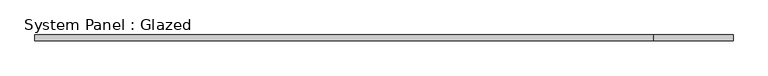
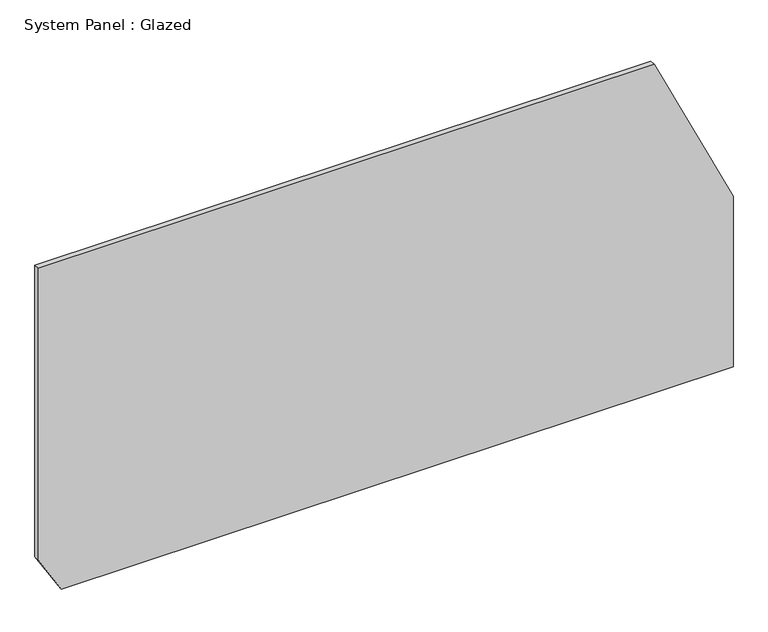
"""IFC4 building model written with IfcOpenShell, lengths in millimetres: plate geometry, System Panel : Glazed."""

import ifcopenshell
import ifcopenshell.guid

model = None  # the IFC model being written
_history = None  # IfcOwnerHistory: only IFC2X3 demands one
_inside = {}  # id of a spatial element -> (the spatial element, [elements in it])
_under = {}  # id of a project, library or spatial element -> (it, [spatial elements below it])
_declared = {}  # id of a project -> (the project, [libraries it declares])
_typed = {}  # id of a type object -> (the type object, [elements of that type])
_made_of = {}  # id of a material, layer set ... -> (it, [elements and type objects made of it])


def new_model(schema):
    """Start an empty IFC model of exactly this schema.

    Asked for "IFC4X3", IfcOpenShell would pick the latest addendum, in which some entities
    have other attributes; the version numbers below select the first issue.
    IFC2X3 requires an IfcOwnerHistory on every rooted entity: one is made here for all.
    """
    global model, _history
    if schema == "IFC4X3":
        model = ifcopenshell.file(schema_version=(4, 3, 0, 0))
    else:
        model = ifcopenshell.file(schema=schema)
    _inside.clear()
    _under.clear()
    _declared.clear()
    _typed.clear()
    _made_of.clear()
    _history = None
    if model.schema == "IFC2X3":
        org = make("IfcOrganization", Name="unknown")
        user = make(
            "IfcPersonAndOrganization",
            ThePerson=make("IfcPerson", FamilyName="unknown"),
            TheOrganization=org,
        )
        app = make(
            "IfcApplication",
            ApplicationDeveloper=org,
            Version="unknown",
            ApplicationFullName="unknown",
            ApplicationIdentifier="unknown",
        )
        _history = make(
            "IfcOwnerHistory",
            OwningUser=user,
            OwningApplication=app,
            ChangeAction="ADDED",
            CreationDate=0,
        )
    return model


def make(cls, **values):
    """One entity of the class cls with the attributes given. An attribute that is None is left unset."""
    return model.create_entity(
        cls, **{name: value for name, value in values.items() if value is not None}
    )


def rooted(cls, **values):
    """An entity with a GlobalId (a new one), such as an element, a storey or a relation."""
    return make(cls, GlobalId=ifcopenshell.guid.new(), OwnerHistory=_history, **values)


def si_unit(unit_type, name, prefix=None):
    """IfcSIUnit, for example si_unit("LENGTHUNIT", "METRE", prefix="MILLI")."""
    return make("IfcSIUnit", UnitType=unit_type, Prefix=prefix, Name=name)


def assignment(units):
    """IfcUnitAssignment: the units of a project."""
    return None if units is None else make("IfcUnitAssignment", Units=units)


def point(xyz):
    """IfcCartesianPoint."""
    return None if xyz is None else make("IfcCartesianPoint", Coordinates=xyz)


def direction(xyz):
    """IfcDirection."""
    return None if xyz is None else make("IfcDirection", DirectionRatios=xyz)


def frame(location, z_axis=None, x_axis=None):
    """IfcAxis2Placement3D, a coordinate frame: its origin and axes. An axis left out is left unset."""
    return make(
        "IfcAxis2Placement3D",
        Location=point(location),
        Axis=direction(z_axis),
        RefDirection=direction(x_axis),
    )


def origin():
    """The frame at (0, 0, 0) with its axes left unset."""
    return frame((0.0, 0.0, 0.0))


def place(relative_to, where):
    """IfcLocalPlacement: puts the frame where relative to a parent placement (None: the world)."""
    return make(
        "IfcLocalPlacement", PlacementRelTo=relative_to, RelativePlacement=where
    )


def context(
    kind, dimensions, precision=None, world=None, true_north=None, identifier=None
):
    """IfcGeometricRepresentationContext, for example the 3D "Model" context."""
    return make(
        "IfcGeometricRepresentationContext",
        ContextIdentifier=identifier,
        ContextType=kind,
        CoordinateSpaceDimension=dimensions,
        Precision=precision,
        WorldCoordinateSystem=world,
        TrueNorth=true_north,
    )


def project(units=None, contexts=None):
    """IfcProject with its units and contexts."""
    return rooted(
        "IfcProject",
        Name="project",
        RepresentationContexts=contexts,
        UnitsInContext=assignment(units),
    )


def spatial(cls, under=None, at=None, **own):
    """A site, building, storey or space (cls), placed at a placement, below another one or the project."""
    s = rooted(cls, ObjectPlacement=at, **own)
    if under is not None:
        _under.setdefault(under.id(), (under, []))[1].append(s)
    return s


def polyline(points):
    """IfcPolyline through the points."""
    return make("IfcPolyline", Points=[point(p) for p in points])


def outline(outer, holes=None, kind="AREA"):
    """IfcArbitraryClosedProfileDef: a profile drawn as a closed curve; with holes, ...WithVoids."""
    if holes is None:
        return make("IfcArbitraryClosedProfileDef", ProfileType=kind, OuterCurve=outer)
    return make(
        "IfcArbitraryProfileDefWithVoids",
        ProfileType=kind,
        OuterCurve=outer,
        InnerCurves=holes,
    )


def extrude(swept, where, along, depth):
    """IfcExtrudedAreaSolid: the profile swept, set in the frame where, extruded along a direction by depth."""
    return make(
        "IfcExtrudedAreaSolid",
        SweptArea=swept,
        Position=where,
        ExtrudedDirection=direction(along),
        Depth=depth,
    )


def shape(context_of_items, identifier, shape_type, items):
    """IfcShapeRepresentation: the items that make up one representation, for example the "Body"."""
    return make(
        "IfcShapeRepresentation",
        ContextOfItems=context_of_items,
        RepresentationIdentifier=identifier,
        RepresentationType=shape_type,
        Items=items,
    )


def source(mapping_origin, context_of_items, identifier, shape_type, items):
    """IfcRepresentationMap: a shape defined once, which mapped items show again and again."""
    return make(
        "IfcRepresentationMap",
        MappingOrigin=mapping_origin,
        MappedRepresentation=shape(context_of_items, identifier, shape_type, items),
    )


def transform(
    local_origin,
    x_axis=None,
    y_axis=None,
    z_axis=None,
    scale=None,
    scale2=None,
    scale3=None,
    uniform=True,
):
    """IfcCartesianTransformationOperator3D, or its non-uniform kind. x_axis, y_axis, z_axis: its Axis1, 2, 3."""
    if uniform:
        return make(
            "IfcCartesianTransformationOperator3D",
            Axis1=direction(x_axis),
            Axis2=direction(y_axis),
            LocalOrigin=point(local_origin),
            Scale=scale,
            Axis3=direction(z_axis),
        )
    return make(
        "IfcCartesianTransformationOperator3DnonUniform",
        Axis1=direction(x_axis),
        Axis2=direction(y_axis),
        LocalOrigin=point(local_origin),
        Scale=scale,
        Axis3=direction(z_axis),
        Scale2=scale2,
        Scale3=scale3,
    )


def mapped(mapping_source, mapping_target):
    """IfcMappedItem: shows the shape of a source again, moved by a transform."""
    return make(
        "IfcMappedItem", MappingSource=mapping_source, MappingTarget=mapping_target
    )


def made_of(thing, what):
    """Note that an element or type object is made of a material, layer set ...; save() writes the relation."""
    if what is not None:
        _made_of.setdefault(what.id(), (what, []))[1].append(thing)
    return thing


def element(
    cls,
    number,
    at=None,
    inside=None,
    cuts=None,
    type_object=None,
    material=None,
    context=None,
    identifier="Body",
    shape_type=None,
    held_by="IfcProductDefinitionShape",
    body=None,
    shapes=None,
    **own,
):
    """One element of the class cls, such as IfcWall. Its Tag is "e" and its number.

    at: its placement. inside: the storey or other place that contains it. cuts: it is an
    opening in that element (IfcRelVoidsElement). A single representation is given by context,
    identifier, shape_type and body (its items); several are given by shapes. held_by: the class
    of the entity that holds the representations. save() writes the other relations.
    """
    e = rooted(cls, Tag="e%d" % number, ObjectPlacement=at, **own)
    if body is not None:
        shapes = [shape(context, identifier, shape_type, body)]
    if shapes is not None:
        e.Representation = make(held_by, Representations=shapes)
    if inside is not None:
        _inside.setdefault(inside.id(), (inside, []))[1].append(e)
    if cuts is not None:
        rooted(
            "IfcRelVoidsElement", RelatingBuildingElement=cuts, RelatedOpeningElement=e
        )
    if type_object is not None:
        _typed.setdefault(type_object.id(), (type_object, []))[1].append(e)
    return made_of(e, material)


def aggregate(whole, parts):
    """IfcRelAggregates: a whole, such as a stair, and the parts it consists of."""
    return rooted("IfcRelAggregates", RelatingObject=whole, RelatedObjects=parts)


def save(model, path):
    """Write the relations noted so far, then the file.

    IfcRelAggregates (storeys below a building ...), IfcRelContainedInSpatialStructure (elements
    in a storey), IfcRelDefinesByType, IfcRelAssociatesMaterial and IfcRelDeclares: one each for
    every whole, place, type object, material and project.
    """
    for whole, parts in _under.values():
        aggregate(whole, parts)
    for where, things in _inside.values():
        rooted(
            "IfcRelContainedInSpatialStructure",
            RelatedElements=things,
            RelatingStructure=where,
        )
    for kind, things in _typed.values():
        rooted("IfcRelDefinesByType", RelatedObjects=things, RelatingType=kind)
    for what, things in _made_of.values():
        rooted("IfcRelAssociatesMaterial", RelatedObjects=things, RelatingMaterial=what)
    for by, libraries in _declared.values():
        rooted("IfcRelDeclares", RelatingContext=by, RelatedDefinitions=libraries)
    model.write(path)


def system_panel_glazed_3905b19f(model_context):
    return source(origin(), model_context, "Body", "SweptSolid", [
        extrude(outline(polyline([(0.0, -1399.9529645), (0.0, 1500.0), (779.2966956, 1500.0), (1500.0, 1159.42413), (1500.0, -1500.0), (167.838939, -1500.0), (0.0, -1399.9529645)])), frame((0.0, 24.5, 0.0), z_axis=(0.0, 1.0, 0.0), x_axis=(0.0, 0.0, 1.0)), (0.0, 0.0, 1.0), 25.0),
    ])


if __name__ == "__main__":
    model = new_model("IFC4")
    model_context = context("Model", 3, world=origin())
    ifc_project = project(units=[si_unit("LENGTHUNIT", "METRE", prefix="MILLI")], contexts=[model_context])
    site = spatial("IfcSite", under=ifc_project)
    building = spatial("IfcBuilding", under=site)
    placement = place(None, origin())
    system_panel_glazed_shape = system_panel_glazed_3905b19f(model_context)
    element("IfcPlate", 1, ObjectType="System Panel : Glazed", at=placement, inside=building, context=model_context, shape_type="MappedRepresentation", body=[
        mapped(system_panel_glazed_shape, transform((0.0, 0.0, 0.0), x_axis=(1.0, 0.0, 0.0), y_axis=(0.0, 1.0, 0.0), z_axis=(0.0, 0.0, 1.0))),
    ])
    save(model, "model.ifc")

# Revit data of these elements
# Type "System Panel : Glazed"
#   Construction Type Id = "GSP4R"
#   Analytic Construction = "1/8 in Pilkington single glazing"
#   Visual Light Transmittance = 0.9
#   Solar Heat Gain Coefficient = 0.86
#   Heat Transfer Coefficient (U) = 6.7069 W/(m²·K)
#   Define Thermal Properties by = 1
# Element 1 (IfcPlate, "System Panel : Glazed")
#   Materials on its faces: "Glass"
# Materials
#   "Glass": class "Glass", colour RGB 0 128 192, transparency 0.9, Description = "Soda Lime Glass", Cost = 0
